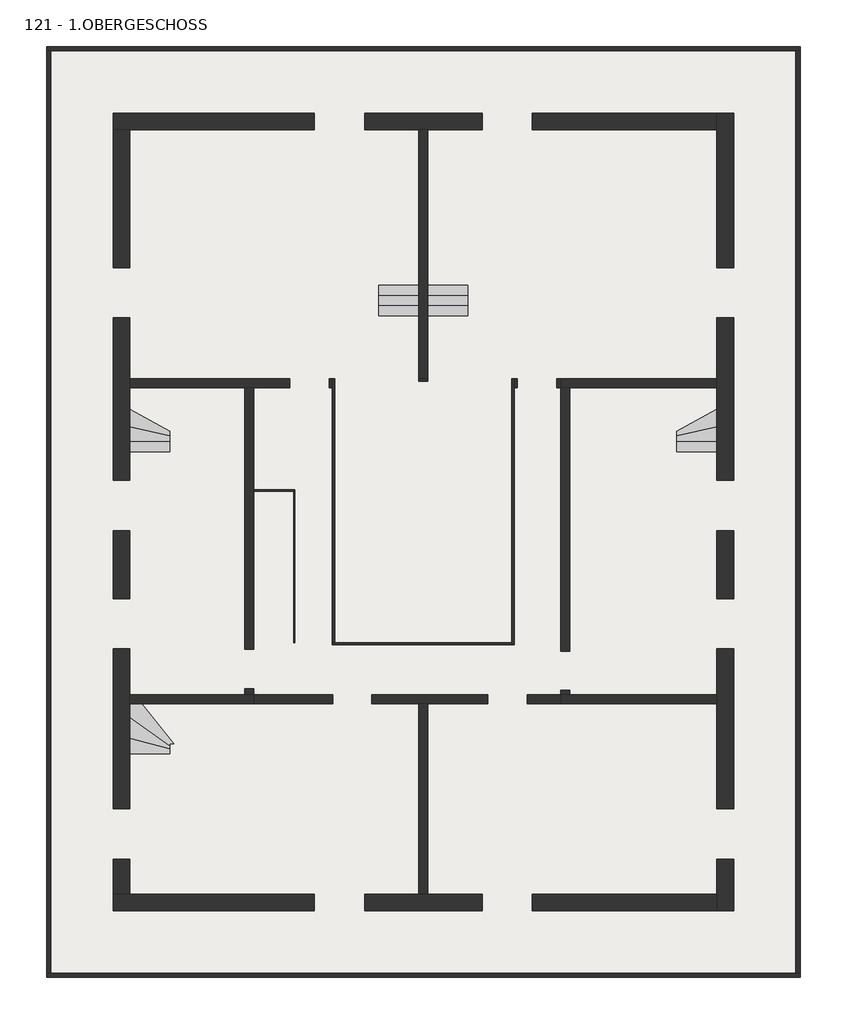
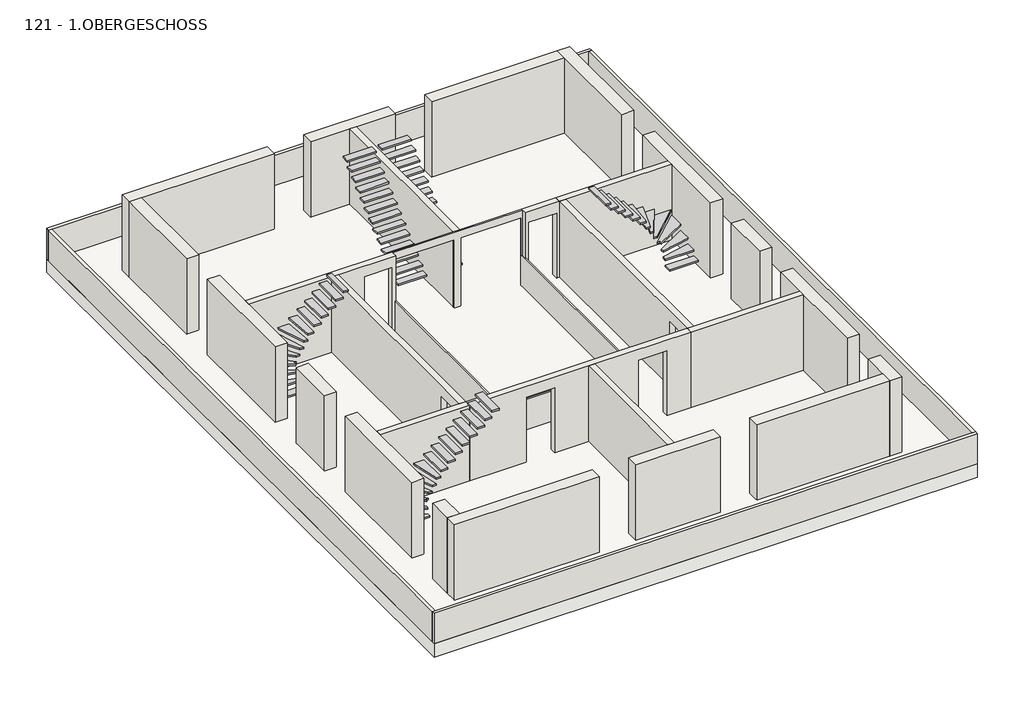
# One storey: 24 walls, 10 stairs, 1 slab.
# Revit data of these elements (continued)
# Room at (3928.317, 16360) mm, phase "New Construction", upper offset 2.500 m, lower offset 0.000 m
#   Export to IFC As = "ifcspace"
#   IfcGUID = "3J0l6V$An1WgW4ojn5k9EU"
#   Comments = ""
#   Number = "36"
#   Name = "Zimmer 6"
#   Abrechnungsart = "m²"
#   Allright_Bauteil_ID = "0121Rau0785066399"
#   Objektname = "Raum"
#   Status = "Neubau"
#   Flächenart_DIN277 = "N"
#   Flächenart_Wohnfläche = "WO"
#   Nutzungsart_Din277 = "NUF"
#   Ortscode_Geschoßbezeichnung = "OG"
#   Raumumschließung = "R"
#   Faktor_DIN277 = 1
#   Faktor_Wohnfläche_Raum = 1
#   BauNVO_Anrechnung_auf_GF = 0
#   BauNVO_Anrechnung_auf_GR = 0
#   Raum unter Treppe (Wohnfl erst ab 2m) = 0
